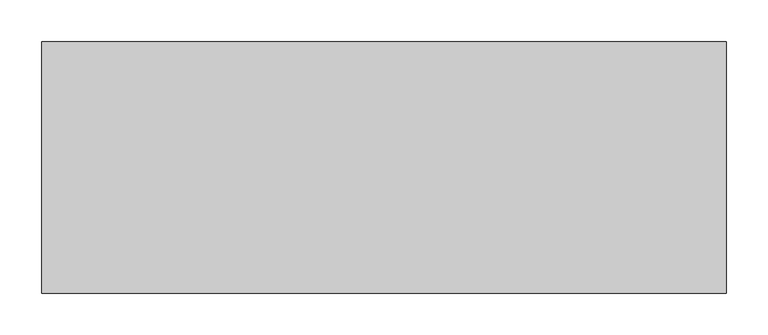
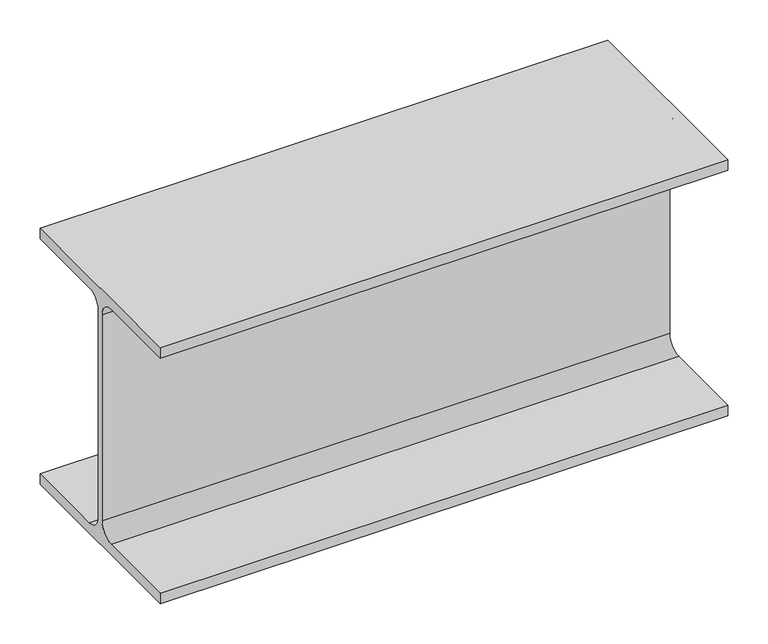
"""IFC4 building model written with IfcOpenShell, lengths in millimetres: beam geometry, 0912_Steel Framing_H-KSD3502 : H_SB_ASB_H-390x300x10x16."""

from ifc_helpers import new_model, si_unit, point, frame, frame_2d, origin, place, context, project, spatial, polyline, circle_curve, trimmed, segment, composite_curve, outline, extrude, source, transform, mapped, element, save


def beam_6b16d095(model_context):
    return source(origin(), model_context, "Body", "SweptSolid", [
        extrude(outline(composite_curve([segment(polyline([(150.0, -179.0), (150.0, -195.0), (-150.0, -195.0), (-150.0, -179.0), (-27.0, -179.0)]), True, "CONTINUOUS"), segment(trimmed(circle_curve(frame_2d((-27.0, -157.0)), 22.0), [point((-27.0, -179.0))], [point((-5.0, -157.0))], True, "CARTESIAN"), True, "CONTINUOUS"), segment(polyline([(-5.0, -157.0), (-5.0, 157.0)]), True, "CONTINUOUS"), segment(trimmed(circle_curve(frame_2d((-27.0, 157.0)), 22.0), [point((-5.0, 157.0))], [point((-27.0, 179.0))], True, "CARTESIAN"), True, "CONTINUOUS"), segment(polyline([(-27.0, 179.0), (-150.0, 179.0), (-150.0, 195.0), (150.0, 195.0), (150.0, 179.0), (27.0, 179.0)]), True, "CONTINUOUS"), segment(trimmed(circle_curve(frame_2d((27.0, 157.0)), 22.0), [point((27.0, 179.0))], [point((5.0, 157.0))], True, "CARTESIAN"), True, "CONTINUOUS"), segment(polyline([(5.0, 157.0), (5.0, -157.0)]), True, "CONTINUOUS"), segment(trimmed(circle_curve(frame_2d((27.0, -157.0)), 22.0), [point((5.0, -157.0))], [point((27.0, -179.0))], True, "CARTESIAN"), True, "CONTINUOUS"), segment(polyline([(27.0, -179.0), (150.0, -179.0)]), True, "CONTINUOUS")], self_intersect=False)), frame((-415.0, 0.0, 0.0), z_axis=(1.0, 0.0, 0.0), x_axis=(0.0, 1.0, 0.0)), (0.0, 0.0, 1.0), 817.2999994),
    ])


if __name__ == "__main__":
    model = new_model("IFC4")
    model_context = context("Model", 3, world=origin())
    ifc_project = project(units=[si_unit("LENGTHUNIT", "METRE", prefix="MILLI")], contexts=[model_context])
    site = spatial("IfcSite", under=ifc_project)
    building = spatial("IfcBuilding", under=site)
    placement = place(None, origin())
    beam_shape = beam_6b16d095(model_context)
    element("IfcBeam", 1, ObjectType="0912_Steel Framing_H-KSD3502 : H_SB_ASB_H-390x300x10x16", at=placement, inside=building, context=model_context, shape_type="MappedRepresentation", body=[
        mapped(beam_shape, transform((0.0, 0.0, 0.0), x_axis=(1.0, 0.0, 0.0), y_axis=(0.0, 1.0, 0.0), z_axis=(0.0, 0.0, 1.0))),
    ])
    save(model, "model.ifc")

# Revit data of these elements
# Type "0912_Steel Framing_H-KSD3502 : H_SB_ASB_H-390x300x10x16"
#   H_WM Code_1 = "S01AA001-00001 | Main Steel Structure Fabrication Work | Shelter/Building | Heavy Steel - Standard (Weight≥90KG/M) | Material: (   )"
#   H_WM Code_2 = "S03AA027-00001 | Main Steel Structure Erection Work | Shelter/Building | Heavy Steel (Weight≥90KG/M) | Material: (   )"
#   H_WM Code_3 = "S01AA010-00001 | Main Steel Structure Fabrication Work | Shelter/Building | Steel Painting/Coating | for Non-Fireproofed Steel Surface, Surface Preparation, Primer, Second & Final Coat | Material: (   )"
#   H_Q'ty Cal Type Tag = "SB-Q2"
#   Width = 30.0 cm
#   Web Thickness = 1.0 cm
#   Web Fillet = 2.2 cm
#   Warping Constant = 2520000.0 cm⁶
#   W = 0
#   Torsional Moment of Inertia = 94.3867 cm⁴
#   Section Area = 136.0 cm²
#   Plastic Modulus weak axis = 733.0 cm³
#   Plastic Modulus strong axis = 2190.0 cm³
#   Perimeter = 1.92 m²/m
#   Nominal Weight = 107.00 kgf/m
#   Moment of Inertia weak axis = 7210.00 cm⁴
#   Moment of Inertia strong axis = 38700.00 cm⁴
#   Height = 39.0 cm
#   Flange Thickness = 1.6 cm
#   Elastic Modulus weak axis = 481.0 cm³
#   Elastic Modulus strong axis = 1980.0 cm³
#   Centroid Vertical = 19.5 cm
#   Centroid Horizontal = 15.0 cm
#   Ix = 387000000
#   Length [instance default] = 1.5240 m
#   Zx = 2190000
#   b = 0.3000 m
#   h = 0.3900 m
#   r = 0.0220 m
#   s = 0.0100 m
#   t = 0.0160 m
#   A = 0.0136 m²
#   Structural Material [instance default] = Steel, 45-345
#   Assembly Code = ""
# Element 1 (IfcBeam, "0912_Steel Framing_H-KSD3502 : H_SB_ASB_H-390x300x10x16")
#   Structural Material = none
# Materials
#   "Steel, 45-345": class "Metal", colour RGB 189 187 185, transparency 0, Description = "Steel 345 MPa", Cost = 0
